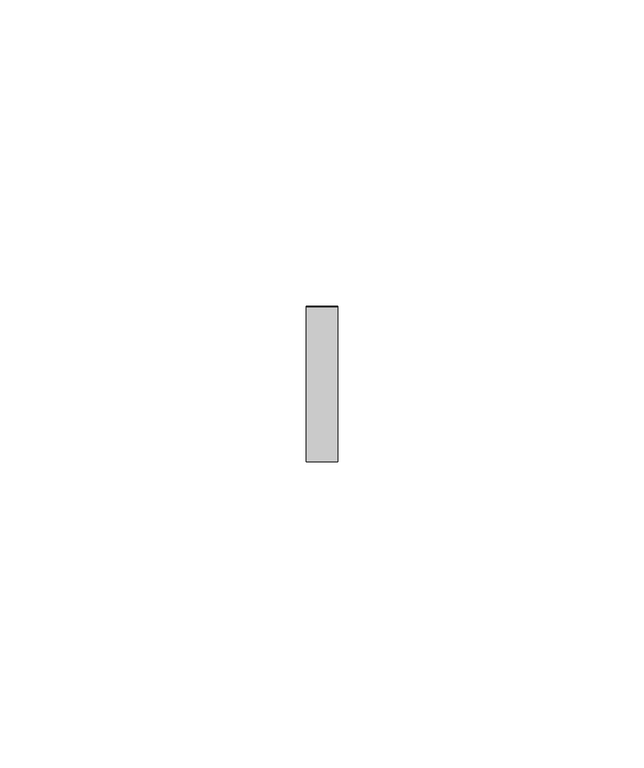
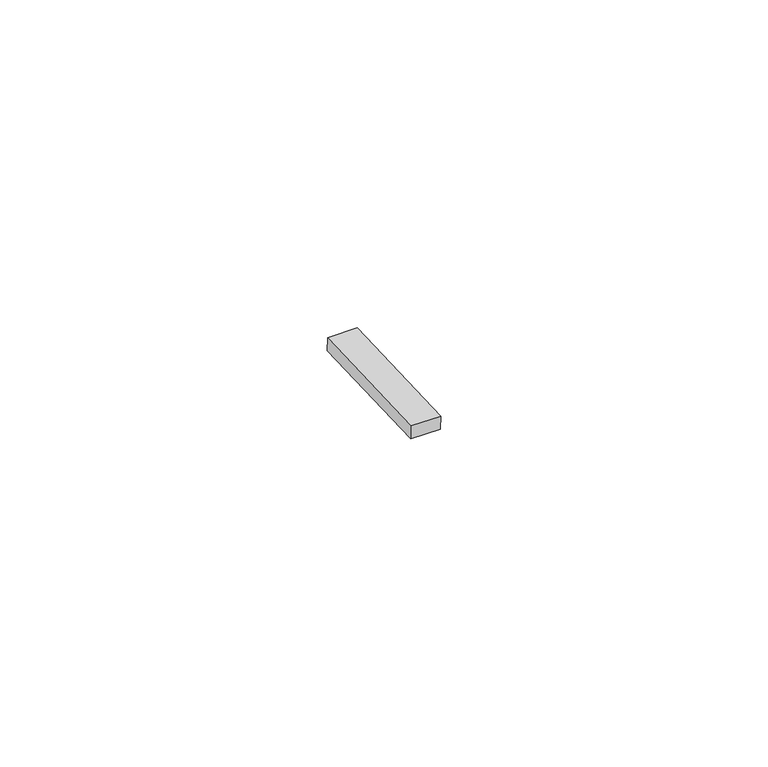
"""IFC4 building model written with IfcOpenShell, lengths in millimetres: proxy geometry, Inner panel:Inner panel:1:Inner panel:1 : Inner panel:Inner panel:300324:2:Inner panel:1:Inner panel:1 : Inner panel:Inner panel:300324:2 : Inner panel:Inner panel:1:Inner panel:1 : Inner panel:Inner panel:300324:300043:127 : Inner panel:Inner panel:1:Inner panel:1 : Inner panel:Inner panel:300324:2:Inner panel:1:Inner panel:1 : Inner panel:Inner panel:300324:2 : Inner panel:Inner panel:1:Inner panel:1 : Inner panel:Inner panel:300324:300043:308120."""

from ifc_helpers import new_model, si_unit, frame, origin, place, context, project, spatial, polyline, outline, extrude, source, transform, mapped, element, save


def generic_models_1bd5f1f2(model_context):
    return source(origin(), model_context, "Body", "SweptSolid", [
        extrude(outline(polyline([(0.0, -25.3999999), (0.0, 0.0), (5.2138089, 0.0), (5.2138089, -25.3999999), (0.0, -25.3999999)])), frame((592717.395117, -577413.7950993, 4016.01903), z_axis=(0.0, -0.041630544712223896, 0.9991330730923502), x_axis=(-1.0, 0.0, 0.0)), (0.0, 0.0, 1.0), 2.4763745),
    ])


if __name__ == "__main__":
    model = new_model("IFC4")
    model_context = context("Model", 3, world=origin())
    ifc_project = project(units=[si_unit("LENGTHUNIT", "METRE", prefix="MILLI")], contexts=[model_context])
    site = spatial("IfcSite", under=ifc_project)
    building = spatial("IfcBuilding", under=site)
    placement = place(None, origin())
    generic_models_shape = generic_models_1bd5f1f2(model_context)
    element("IfcBuildingElementProxy", 1, Name="Inner panel:Inner panel:1:Inner panel:1 : Inner panel:Inner panel:300324:2:Inner panel:1:Inner panel:1 : Inner panel:Inner panel:300324:2 : Inner panel:Inner panel:1:Inner panel:1 : Inner panel:Inner panel:300324:300043:127 : Inner panel:Inner panel:1:Inner panel:1 : Inner panel:Inner panel:300324:2:Inner panel:1:Inner panel:1 : Inner panel:Inner panel:300324:2 : Inner panel:Inner panel:1:Inner panel:1 : Inner panel:Inner panel:300324:300043:308120", ObjectType="Inner panel:Inner panel:1:Inner panel:1 : Inner panel:Inner panel:300324:2:Inner panel:1:Inner panel:1 : Inner panel:Inner panel:300324:2 : Inner panel:Inner panel:1:Inner panel:1 : Inner panel:Inner panel:300324:300043:127 : Inner panel:Inner panel:1:Inner panel:1 : Inner panel:Inner panel:300324:2:Inner panel:1:Inner panel:1 : Inner panel:Inner panel:300324:2 : Inner panel:Inner panel:1:Inner panel:1 : Inner panel:Inner panel:300324:300043:308120", at=placement, inside=building, context=model_context, shape_type="MappedRepresentation", body=[
        mapped(generic_models_shape, transform((0.0, 0.0, 0.0), x_axis=(1.0, 0.0, 0.0), y_axis=(0.0, 1.0, 0.0), z_axis=(0.0, 0.0, 1.0))),
    ])
    save(model, "model.ifc")

# Revit data of these elements
# Type "Inner panel:Inner panel:1:Inner panel:1 : Inner panel:Inner panel:300324:2:Inner panel:1:Inner panel:1 : Inner panel:Inner panel:300324:2 : Inner panel:Inner panel:1:Inner panel:1 : Inner panel:Inner panel:300324:300043:127 : Inner panel:Inner panel:1:Inner panel:1 : Inner panel:Inner panel:300324:2:Inner panel:1:Inner panel:1 : Inner panel:Inner panel:300324:2 : Inner panel:Inner panel:1:Inner panel:1 : Inner panel:Inner panel:300324:300043:308120"
#   NameOverride = "Inner panel:Inner panel:1:Inner panel:1 : Inner panel:Inner panel:300324:2:Inner panel:1:Inner panel:1 : Inner panel:Inner panel:300324:2 : Inner panel:Inner panel:1:Inner panel:1 : Inner panel:Inner panel:300324:300043:308120"
#   ObjectTypeOverride = "Inner panel:1:Inner panel:1 : Inner panel:Inner panel:300324:2 : Inner panel:Inner panel:1:Inner panel:1 : Inner panel:Inner panel:300324:300043"
#   Reference = "Inner panel"
#   Tag = "308120"
# Element 1 (IfcBuildingElementProxy, "Inner panel:Inner panel:1:Inner panel:1 : Inner panel:Inner panel:300324:2:Inner panel:1:Inner panel:1 : Inner panel:Inner panel:300324:2 : Inner panel:Inner panel:1:Inner panel:1 : Inner panel:Inner panel:300324:300043:127 : Inner panel:Inner panel:1:Inner panel:1 : Inner panel:Inner panel:300324:2:Inner panel:1:Inner panel:1 : Inner panel:Inner panel:300324:2 : Inner panel:Inner panel:1:Inner panel:1 : Inner panel:Inner panel:300324:300043:308120")
#   Materials on its faces: "AT CLIP - 1\" WIDE NON ABSORBENT, WEATHER-RESISTANT NEOPRENE/EPDM/SBR FOAM"
# Materials
#   "AT CLIP - 1\" WIDE NON ABSORBENT, WEATHER-RESISTANT NEOPRENE/EPDM/SBR FOAM": class "Generic", colour RGB 85 85 85, transparency 0, Cost = 0
